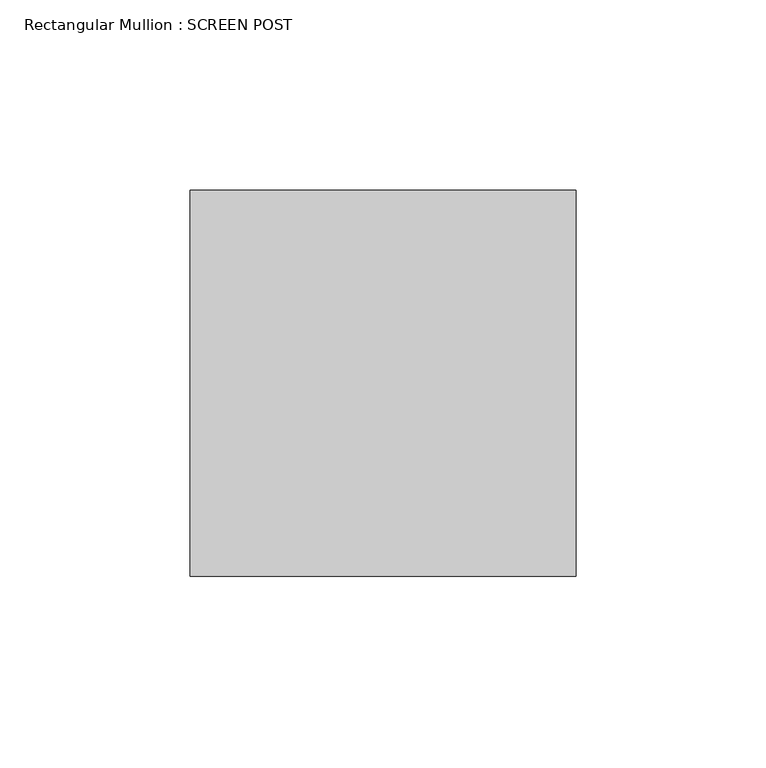
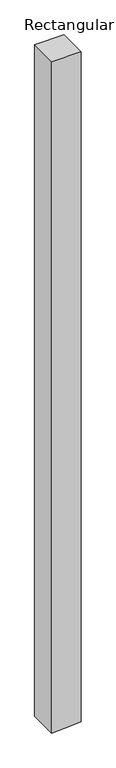
"""IFC4 building model written with IfcOpenShell, lengths in millimetres: member geometry, Rectangular Mullion : SCREEN POST."""

import ifcopenshell
import ifcopenshell.guid

model = None  # the IFC model being written
_history = None  # IfcOwnerHistory: only IFC2X3 demands one
_inside = {}  # id of a spatial element -> (the spatial element, [elements in it])
_under = {}  # id of a project, library or spatial element -> (it, [spatial elements below it])
_declared = {}  # id of a project -> (the project, [libraries it declares])
_typed = {}  # id of a type object -> (the type object, [elements of that type])
_made_of = {}  # id of a material, layer set ... -> (it, [elements and type objects made of it])


def new_model(schema):
    """Start an empty IFC model of exactly this schema.

    Asked for "IFC4X3", IfcOpenShell would pick the latest addendum, in which some entities
    have other attributes; the version numbers below select the first issue.
    IFC2X3 requires an IfcOwnerHistory on every rooted entity: one is made here for all.
    """
    global model, _history
    if schema == "IFC4X3":
        model = ifcopenshell.file(schema_version=(4, 3, 0, 0))
    else:
        model = ifcopenshell.file(schema=schema)
    _inside.clear()
    _under.clear()
    _declared.clear()
    _typed.clear()
    _made_of.clear()
    _history = None
    if model.schema == "IFC2X3":
        org = make("IfcOrganization", Name="unknown")
        user = make(
            "IfcPersonAndOrganization",
            ThePerson=make("IfcPerson", FamilyName="unknown"),
            TheOrganization=org,
        )
        app = make(
            "IfcApplication",
            ApplicationDeveloper=org,
            Version="unknown",
            ApplicationFullName="unknown",
            ApplicationIdentifier="unknown",
        )
        _history = make(
            "IfcOwnerHistory",
            OwningUser=user,
            OwningApplication=app,
            ChangeAction="ADDED",
            CreationDate=0,
        )
    return model


def make(cls, **values):
    """One entity of the class cls with the attributes given. An attribute that is None is left unset."""
    return model.create_entity(
        cls, **{name: value for name, value in values.items() if value is not None}
    )


def rooted(cls, **values):
    """An entity with a GlobalId (a new one), such as an element, a storey or a relation."""
    return make(cls, GlobalId=ifcopenshell.guid.new(), OwnerHistory=_history, **values)


def si_unit(unit_type, name, prefix=None):
    """IfcSIUnit, for example si_unit("LENGTHUNIT", "METRE", prefix="MILLI")."""
    return make("IfcSIUnit", UnitType=unit_type, Prefix=prefix, Name=name)


def assignment(units):
    """IfcUnitAssignment: the units of a project."""
    return None if units is None else make("IfcUnitAssignment", Units=units)


def point(xyz):
    """IfcCartesianPoint."""
    return None if xyz is None else make("IfcCartesianPoint", Coordinates=xyz)


def direction(xyz):
    """IfcDirection."""
    return None if xyz is None else make("IfcDirection", DirectionRatios=xyz)


def frame(location, z_axis=None, x_axis=None):
    """IfcAxis2Placement3D, a coordinate frame: its origin and axes. An axis left out is left unset."""
    return make(
        "IfcAxis2Placement3D",
        Location=point(location),
        Axis=direction(z_axis),
        RefDirection=direction(x_axis),
    )


def origin():
    """The frame at (0, 0, 0) with its axes left unset."""
    return frame((0.0, 0.0, 0.0))


def place(relative_to, where):
    """IfcLocalPlacement: puts the frame where relative to a parent placement (None: the world)."""
    return make(
        "IfcLocalPlacement", PlacementRelTo=relative_to, RelativePlacement=where
    )


def context(
    kind, dimensions, precision=None, world=None, true_north=None, identifier=None
):
    """IfcGeometricRepresentationContext, for example the 3D "Model" context."""
    return make(
        "IfcGeometricRepresentationContext",
        ContextIdentifier=identifier,
        ContextType=kind,
        CoordinateSpaceDimension=dimensions,
        Precision=precision,
        WorldCoordinateSystem=world,
        TrueNorth=true_north,
    )


def project(units=None, contexts=None):
    """IfcProject with its units and contexts."""
    return rooted(
        "IfcProject",
        Name="project",
        RepresentationContexts=contexts,
        UnitsInContext=assignment(units),
    )


def spatial(cls, under=None, at=None, **own):
    """A site, building, storey or space (cls), placed at a placement, below another one or the project."""
    s = rooted(cls, ObjectPlacement=at, **own)
    if under is not None:
        _under.setdefault(under.id(), (under, []))[1].append(s)
    return s


def polyline(points):
    """IfcPolyline through the points."""
    return make("IfcPolyline", Points=[point(p) for p in points])


def outline(outer, holes=None, kind="AREA"):
    """IfcArbitraryClosedProfileDef: a profile drawn as a closed curve; with holes, ...WithVoids."""
    if holes is None:
        return make("IfcArbitraryClosedProfileDef", ProfileType=kind, OuterCurve=outer)
    return make(
        "IfcArbitraryProfileDefWithVoids",
        ProfileType=kind,
        OuterCurve=outer,
        InnerCurves=holes,
    )


def extrude(swept, where, along, depth):
    """IfcExtrudedAreaSolid: the profile swept, set in the frame where, extruded along a direction by depth."""
    return make(
        "IfcExtrudedAreaSolid",
        SweptArea=swept,
        Position=where,
        ExtrudedDirection=direction(along),
        Depth=depth,
    )


def shape(context_of_items, identifier, shape_type, items):
    """IfcShapeRepresentation: the items that make up one representation, for example the "Body"."""
    return make(
        "IfcShapeRepresentation",
        ContextOfItems=context_of_items,
        RepresentationIdentifier=identifier,
        RepresentationType=shape_type,
        Items=items,
    )


def source(mapping_origin, context_of_items, identifier, shape_type, items):
    """IfcRepresentationMap: a shape defined once, which mapped items show again and again."""
    return make(
        "IfcRepresentationMap",
        MappingOrigin=mapping_origin,
        MappedRepresentation=shape(context_of_items, identifier, shape_type, items),
    )


def transform(
    local_origin,
    x_axis=None,
    y_axis=None,
    z_axis=None,
    scale=None,
    scale2=None,
    scale3=None,
    uniform=True,
):
    """IfcCartesianTransformationOperator3D, or its non-uniform kind. x_axis, y_axis, z_axis: its Axis1, 2, 3."""
    if uniform:
        return make(
            "IfcCartesianTransformationOperator3D",
            Axis1=direction(x_axis),
            Axis2=direction(y_axis),
            LocalOrigin=point(local_origin),
            Scale=scale,
            Axis3=direction(z_axis),
        )
    return make(
        "IfcCartesianTransformationOperator3DnonUniform",
        Axis1=direction(x_axis),
        Axis2=direction(y_axis),
        LocalOrigin=point(local_origin),
        Scale=scale,
        Axis3=direction(z_axis),
        Scale2=scale2,
        Scale3=scale3,
    )


def mapped(mapping_source, mapping_target):
    """IfcMappedItem: shows the shape of a source again, moved by a transform."""
    return make(
        "IfcMappedItem", MappingSource=mapping_source, MappingTarget=mapping_target
    )


def made_of(thing, what):
    """Note that an element or type object is made of a material, layer set ...; save() writes the relation."""
    if what is not None:
        _made_of.setdefault(what.id(), (what, []))[1].append(thing)
    return thing


def element(
    cls,
    number,
    at=None,
    inside=None,
    cuts=None,
    type_object=None,
    material=None,
    context=None,
    identifier="Body",
    shape_type=None,
    held_by="IfcProductDefinitionShape",
    body=None,
    shapes=None,
    **own,
):
    """One element of the class cls, such as IfcWall. Its Tag is "e" and its number.

    at: its placement. inside: the storey or other place that contains it. cuts: it is an
    opening in that element (IfcRelVoidsElement). A single representation is given by context,
    identifier, shape_type and body (its items); several are given by shapes. held_by: the class
    of the entity that holds the representations. save() writes the other relations.
    """
    e = rooted(cls, Tag="e%d" % number, ObjectPlacement=at, **own)
    if body is not None:
        shapes = [shape(context, identifier, shape_type, body)]
    if shapes is not None:
        e.Representation = make(held_by, Representations=shapes)
    if inside is not None:
        _inside.setdefault(inside.id(), (inside, []))[1].append(e)
    if cuts is not None:
        rooted(
            "IfcRelVoidsElement", RelatingBuildingElement=cuts, RelatedOpeningElement=e
        )
    if type_object is not None:
        _typed.setdefault(type_object.id(), (type_object, []))[1].append(e)
    return made_of(e, material)


def aggregate(whole, parts):
    """IfcRelAggregates: a whole, such as a stair, and the parts it consists of."""
    return rooted("IfcRelAggregates", RelatingObject=whole, RelatedObjects=parts)


def save(model, path):
    """Write the relations noted so far, then the file.

    IfcRelAggregates (storeys below a building ...), IfcRelContainedInSpatialStructure (elements
    in a storey), IfcRelDefinesByType, IfcRelAssociatesMaterial and IfcRelDeclares: one each for
    every whole, place, type object, material and project.
    """
    for whole, parts in _under.values():
        aggregate(whole, parts)
    for where, things in _inside.values():
        rooted(
            "IfcRelContainedInSpatialStructure",
            RelatedElements=things,
            RelatingStructure=where,
        )
    for kind, things in _typed.values():
        rooted("IfcRelDefinesByType", RelatedObjects=things, RelatingType=kind)
    for what, things in _made_of.values():
        rooted("IfcRelAssociatesMaterial", RelatedObjects=things, RelatingMaterial=what)
    for by, libraries in _declared.values():
        rooted("IfcRelDeclares", RelatingContext=by, RelatedDefinitions=libraries)
    model.write(path)


def rectangular_mullion_screen_post_553c1fba(model_context):
    return source(origin(), model_context, "Body", "SweptSolid", [
        extrude(outline(polyline([(0.0, 50.8), (0.0, -50.8), (-2444.9237674, -50.8), (-2442.1405632, -6.3490391), (-2438.5622953, 50.8), (0.0, 50.8)])), frame((0.0, -50.8, 0.0), z_axis=(0.0, 1.0, 0.0), x_axis=(0.0, 0.0, 1.0)), (0.0, 0.0, 1.0), 101.6),
    ])


if __name__ == "__main__":
    model = new_model("IFC4")
    model_context = context("Model", 3, world=origin())
    ifc_project = project(units=[si_unit("LENGTHUNIT", "METRE", prefix="MILLI")], contexts=[model_context])
    site = spatial("IfcSite", under=ifc_project)
    building = spatial("IfcBuilding", under=site)
    placement = place(None, origin())
    rectangular_mullion_screen_post_shape = rectangular_mullion_screen_post_553c1fba(model_context)
    element("IfcMember", 1, ObjectType="Rectangular Mullion : SCREEN POST", at=placement, inside=building, context=model_context, shape_type="MappedRepresentation", body=[
        mapped(rectangular_mullion_screen_post_shape, transform((0.0, 0.0, 0.0), x_axis=(1.0, 0.0, 0.0), y_axis=(0.0, 1.0, 0.0), z_axis=(0.0, 0.0, 1.0))),
    ])
    save(model, "model.ifc")

# Revit data of these elements
# Type "Rectangular Mullion : SCREEN POST"
#   built-in parameter 1007304 = 0.333333 (stored number, unit not read)
#   built-in parameter 1007301 = 0.166667 (stored number, unit not read)
#   built-in parameter 1007300 = 0.166667 (stored number, unit not read)
# Element 1 (IfcMember, "Rectangular Mullion : SCREEN POST")
#   Materials on its faces: "GLULAMS COLUMNS\n(PRESSURE TREATED W/ PENTA IN SOLVENT) (EXTERIOR STAIN: PENOFIN VERDE EXT. STAIN - COLOR: CEDAR)"
# Materials
#   "GLULAMS COLUMNS\n(PRESSURE TREATED W/ PENTA IN SOLVENT) (EXTERIOR STAIN: PENOFIN VERDE EXT. STAIN - COLOR: CEDAR)": class "Wood", colour RGB 164 134 123, transparency 0, Description = "Pinus Echinata", Cost = 0
